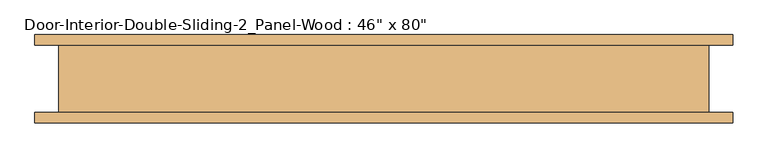
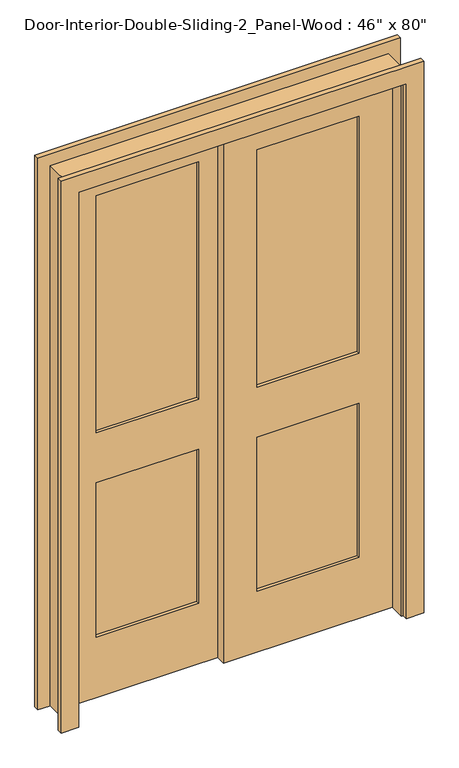
"""IFC4 building model written with IfcOpenShell, lengths in millimetres: door geometry."""

import ifcopenshell
import ifcopenshell.guid

model = None  # the IFC model being written
_history = None  # IfcOwnerHistory: only IFC2X3 demands one
_inside = {}  # id of a spatial element -> (the spatial element, [elements in it])
_under = {}  # id of a project, library or spatial element -> (it, [spatial elements below it])
_declared = {}  # id of a project -> (the project, [libraries it declares])
_typed = {}  # id of a type object -> (the type object, [elements of that type])
_made_of = {}  # id of a material, layer set ... -> (it, [elements and type objects made of it])


def new_model(schema):
    """Start an empty IFC model of exactly this schema.

    Asked for "IFC4X3", IfcOpenShell would pick the latest addendum, in which some entities
    have other attributes; the version numbers below select the first issue.
    IFC2X3 requires an IfcOwnerHistory on every rooted entity: one is made here for all.
    """
    global model, _history
    if schema == "IFC4X3":
        model = ifcopenshell.file(schema_version=(4, 3, 0, 0))
    else:
        model = ifcopenshell.file(schema=schema)
    _inside.clear()
    _under.clear()
    _declared.clear()
    _typed.clear()
    _made_of.clear()
    _history = None
    if model.schema == "IFC2X3":
        org = make("IfcOrganization", Name="unknown")
        user = make(
            "IfcPersonAndOrganization",
            ThePerson=make("IfcPerson", FamilyName="unknown"),
            TheOrganization=org,
        )
        app = make(
            "IfcApplication",
            ApplicationDeveloper=org,
            Version="unknown",
            ApplicationFullName="unknown",
            ApplicationIdentifier="unknown",
        )
        _history = make(
            "IfcOwnerHistory",
            OwningUser=user,
            OwningApplication=app,
            ChangeAction="ADDED",
            CreationDate=0,
        )
    return model


def make(cls, **values):
    """One entity of the class cls with the attributes given. An attribute that is None is left unset."""
    return model.create_entity(
        cls, **{name: value for name, value in values.items() if value is not None}
    )


def rooted(cls, **values):
    """An entity with a GlobalId (a new one), such as an element, a storey or a relation."""
    return make(cls, GlobalId=ifcopenshell.guid.new(), OwnerHistory=_history, **values)


def si_unit(unit_type, name, prefix=None):
    """IfcSIUnit, for example si_unit("LENGTHUNIT", "METRE", prefix="MILLI")."""
    return make("IfcSIUnit", UnitType=unit_type, Prefix=prefix, Name=name)


def assignment(units):
    """IfcUnitAssignment: the units of a project."""
    return None if units is None else make("IfcUnitAssignment", Units=units)


def point(xyz):
    """IfcCartesianPoint."""
    return None if xyz is None else make("IfcCartesianPoint", Coordinates=xyz)


def direction(xyz):
    """IfcDirection."""
    return None if xyz is None else make("IfcDirection", DirectionRatios=xyz)


def frame(location, z_axis=None, x_axis=None):
    """IfcAxis2Placement3D, a coordinate frame: its origin and axes. An axis left out is left unset."""
    return make(
        "IfcAxis2Placement3D",
        Location=point(location),
        Axis=direction(z_axis),
        RefDirection=direction(x_axis),
    )


def origin():
    """The frame at (0, 0, 0) with its axes left unset."""
    return frame((0.0, 0.0, 0.0))


def place(relative_to, where):
    """IfcLocalPlacement: puts the frame where relative to a parent placement (None: the world)."""
    return make(
        "IfcLocalPlacement", PlacementRelTo=relative_to, RelativePlacement=where
    )


def context(
    kind, dimensions, precision=None, world=None, true_north=None, identifier=None
):
    """IfcGeometricRepresentationContext, for example the 3D "Model" context."""
    return make(
        "IfcGeometricRepresentationContext",
        ContextIdentifier=identifier,
        ContextType=kind,
        CoordinateSpaceDimension=dimensions,
        Precision=precision,
        WorldCoordinateSystem=world,
        TrueNorth=true_north,
    )


def project(units=None, contexts=None):
    """IfcProject with its units and contexts."""
    return rooted(
        "IfcProject",
        Name="project",
        RepresentationContexts=contexts,
        UnitsInContext=assignment(units),
    )


def spatial(cls, under=None, at=None, **own):
    """A site, building, storey or space (cls), placed at a placement, below another one or the project."""
    s = rooted(cls, ObjectPlacement=at, **own)
    if under is not None:
        _under.setdefault(under.id(), (under, []))[1].append(s)
    return s


def polyline(points):
    """IfcPolyline through the points."""
    return make("IfcPolyline", Points=[point(p) for p in points])


def outline(outer, holes=None, kind="AREA"):
    """IfcArbitraryClosedProfileDef: a profile drawn as a closed curve; with holes, ...WithVoids."""
    if holes is None:
        return make("IfcArbitraryClosedProfileDef", ProfileType=kind, OuterCurve=outer)
    return make(
        "IfcArbitraryProfileDefWithVoids",
        ProfileType=kind,
        OuterCurve=outer,
        InnerCurves=holes,
    )


def extrude(swept, where, along, depth):
    """IfcExtrudedAreaSolid: the profile swept, set in the frame where, extruded along a direction by depth."""
    return make(
        "IfcExtrudedAreaSolid",
        SweptArea=swept,
        Position=where,
        ExtrudedDirection=direction(along),
        Depth=depth,
    )


def shape(context_of_items, identifier, shape_type, items):
    """IfcShapeRepresentation: the items that make up one representation, for example the "Body"."""
    return make(
        "IfcShapeRepresentation",
        ContextOfItems=context_of_items,
        RepresentationIdentifier=identifier,
        RepresentationType=shape_type,
        Items=items,
    )


def source(mapping_origin, context_of_items, identifier, shape_type, items):
    """IfcRepresentationMap: a shape defined once, which mapped items show again and again."""
    return make(
        "IfcRepresentationMap",
        MappingOrigin=mapping_origin,
        MappedRepresentation=shape(context_of_items, identifier, shape_type, items),
    )


def transform(
    local_origin,
    x_axis=None,
    y_axis=None,
    z_axis=None,
    scale=None,
    scale2=None,
    scale3=None,
    uniform=True,
):
    """IfcCartesianTransformationOperator3D, or its non-uniform kind. x_axis, y_axis, z_axis: its Axis1, 2, 3."""
    if uniform:
        return make(
            "IfcCartesianTransformationOperator3D",
            Axis1=direction(x_axis),
            Axis2=direction(y_axis),
            LocalOrigin=point(local_origin),
            Scale=scale,
            Axis3=direction(z_axis),
        )
    return make(
        "IfcCartesianTransformationOperator3DnonUniform",
        Axis1=direction(x_axis),
        Axis2=direction(y_axis),
        LocalOrigin=point(local_origin),
        Scale=scale,
        Axis3=direction(z_axis),
        Scale2=scale2,
        Scale3=scale3,
    )


def mapped(mapping_source, mapping_target):
    """IfcMappedItem: shows the shape of a source again, moved by a transform."""
    return make(
        "IfcMappedItem", MappingSource=mapping_source, MappingTarget=mapping_target
    )


def made_of(thing, what):
    """Note that an element or type object is made of a material, layer set ...; save() writes the relation."""
    if what is not None:
        _made_of.setdefault(what.id(), (what, []))[1].append(thing)
    return thing


def element(
    cls,
    number,
    at=None,
    inside=None,
    cuts=None,
    type_object=None,
    material=None,
    context=None,
    identifier="Body",
    shape_type=None,
    held_by="IfcProductDefinitionShape",
    body=None,
    shapes=None,
    **own,
):
    """One element of the class cls, such as IfcWall. Its Tag is "e" and its number.

    at: its placement. inside: the storey or other place that contains it. cuts: it is an
    opening in that element (IfcRelVoidsElement). A single representation is given by context,
    identifier, shape_type and body (its items); several are given by shapes. held_by: the class
    of the entity that holds the representations. save() writes the other relations.
    """
    e = rooted(cls, Tag="e%d" % number, ObjectPlacement=at, **own)
    if body is not None:
        shapes = [shape(context, identifier, shape_type, body)]
    if shapes is not None:
        e.Representation = make(held_by, Representations=shapes)
    if inside is not None:
        _inside.setdefault(inside.id(), (inside, []))[1].append(e)
    if cuts is not None:
        rooted(
            "IfcRelVoidsElement", RelatingBuildingElement=cuts, RelatedOpeningElement=e
        )
    if type_object is not None:
        _typed.setdefault(type_object.id(), (type_object, []))[1].append(e)
    return made_of(e, material)


def aggregate(whole, parts):
    """IfcRelAggregates: a whole, such as a stair, and the parts it consists of."""
    return rooted("IfcRelAggregates", RelatingObject=whole, RelatedObjects=parts)


def save(model, path):
    """Write the relations noted so far, then the file.

    IfcRelAggregates (storeys below a building ...), IfcRelContainedInSpatialStructure (elements
    in a storey), IfcRelDefinesByType, IfcRelAssociatesMaterial and IfcRelDeclares: one each for
    every whole, place, type object, material and project.
    """
    for whole, parts in _under.values():
        aggregate(whole, parts)
    for where, things in _inside.values():
        rooted(
            "IfcRelContainedInSpatialStructure",
            RelatedElements=things,
            RelatingStructure=where,
        )
    for kind, things in _typed.values():
        rooted("IfcRelDefinesByType", RelatedObjects=things, RelatingType=kind)
    for what, things in _made_of.values():
        rooted("IfcRelAssociatesMaterial", RelatedObjects=things, RelatingMaterial=what)
    for by, libraries in _declared.values():
        rooted("IfcRelDeclares", RelatingContext=by, RelatedDefinitions=libraries)
    model.write(path)


def door_0fd0fe05(model_context):
    return source(origin(), model_context, "Body", "SweptSolid", [
        extrude(outline(polyline([(463.55, 2.1166667), (95.25, 2.1166667), (95.25, 13.7583333), (463.55, 13.7583333), (463.55, 2.1166667)])), frame((0.0, 0.0, 1009.65), z_axis=(0.0, 0.0, 1.0), x_axis=(1.0, 0.0, 0.0)), (0.0, 0.0, 1.0), 903.2875),
        extrude(outline(polyline([(463.55, 2.1166667), (95.25, 2.1166667), (95.25, 13.7583333), (463.55, 13.7583333), (463.55, 2.1166667)])), frame((0.0, 0.0, 231.775), z_axis=(0.0, 0.0, 1.0), x_axis=(1.0, 0.0, 0.0)), (0.0, 0.0, 1.0), 587.375),
        extrude(outline(polyline([(2032.0, -25.4), (0.0, -25.4), (0.0, 584.2), (2032.0, 584.2), (2032.0, -25.4)]), holes=[polyline([(1912.9375, 95.25), (1912.9375, 463.55), (1009.65, 463.55), (1009.65, 95.25), (1912.9375, 95.25)]), polyline([(819.15, 95.25), (819.15, 463.55), (231.775, 463.55), (231.775, 95.25), (819.15, 95.25)])]), frame((0.0, -9.525, 0.0), z_axis=(0.0, 1.0, 0.0), x_axis=(0.0, 0.0, 1.0)), (0.0, 0.0, 1.0), 34.925),
        extrude(outline(polyline([(-95.25, 37.0416667), (-463.55, 37.0416667), (-463.55, 48.6833333), (-95.25, 48.6833333), (-95.25, 37.0416667)])), frame((0.0, 0.0, 1009.65), z_axis=(0.0, 0.0, 1.0), x_axis=(1.0, 0.0, 0.0)), (0.0, 0.0, 1.0), 903.2875),
        extrude(outline(polyline([(-95.25, 37.0416667), (-463.55, 37.0416667), (-463.55, 48.6833333), (-95.25, 48.6833333), (-95.25, 37.0416667)])), frame((0.0, 0.0, 231.775), z_axis=(0.0, 0.0, 1.0), x_axis=(1.0, 0.0, 0.0)), (0.0, 0.0, 1.0), 587.375),
        extrude(outline(polyline([(2032.0, -584.2), (0.0, -584.2), (0.0, 25.4), (2032.0, 25.4), (2032.0, -584.2)]), holes=[polyline([(1912.9375, -463.55), (1912.9375, -95.25), (1009.65, -95.25), (1009.65, -463.55), (1912.9375, -463.55)]), polyline([(819.15, -463.55), (819.15, -95.25), (231.775, -95.25), (231.775, -463.55), (819.15, -463.55)])]), frame((0.0, 25.4, 0.0), z_axis=(0.0, 1.0, 0.0), x_axis=(0.0, 0.0, 1.0)), (0.0, 0.0, 1.0), 34.925),
        extrude(outline(polyline([(0.0, 584.2), (0.0, 609.6), (2057.4, 609.6), (2057.4, -609.6), (0.0, -609.6), (0.0, -584.2), (2032.0, -584.2), (2032.0, 584.2), (0.0, 584.2)])), frame((0.0, -66.675, 0.0), z_axis=(0.0, 1.0, 0.0), x_axis=(0.0, 0.0, 1.0)), (0.0, 0.0, 1.0), 127.0),
        extrude(outline(polyline([(0.0, 590.55), (0.0, 654.05), (2101.85, 654.05), (2101.85, -654.05), (0.0, -654.05), (0.0, -590.55), (2038.35, -590.55), (2038.35, 590.55), (0.0, 590.55)])), frame((0.0, -85.725, 0.0), z_axis=(0.0, 1.0, 0.0), x_axis=(0.0, 0.0, 1.0)), (0.0, 0.0, 1.0), 19.05),
        extrude(outline(polyline([(0.0, 590.55), (0.0, 654.05), (2101.85, 654.05), (2101.85, -654.05), (0.0, -654.05), (0.0, -590.55), (2038.35, -590.55), (2038.35, 590.55), (0.0, 590.55)])), frame((0.0, 60.325, 0.0), z_axis=(0.0, 1.0, 0.0), x_axis=(0.0, 0.0, 1.0)), (0.0, 0.0, 1.0), 19.05),
    ])


if __name__ == "__main__":
    model = new_model("IFC4")
    model_context = context("Model", 3, world=origin())
    ifc_project = project(units=[si_unit("LENGTHUNIT", "METRE", prefix="MILLI")], contexts=[model_context])
    site = spatial("IfcSite", under=ifc_project)
    building = spatial("IfcBuilding", under=site)
    placement = place(None, origin())
    door_shape = door_0fd0fe05(model_context)
    element("IfcDoor", 1, ObjectType="Door-Interior-Double-Sliding-2_Panel-Wood : 46\" x 80\"", at=placement, inside=building, context=model_context, shape_type="MappedRepresentation", body=[
        mapped(door_shape, transform((0.0, 0.0, 0.0), x_axis=(1.0, 0.0, 0.0), y_axis=(0.0, 1.0, 0.0), z_axis=(0.0, 0.0, 1.0))),
    ])
    save(model, "model.ifc")

# Revit data of these elements
# Type "Door-Interior-Double-Sliding-2_Panel-Wood : 46\" x 80\""
#   Type Mark = "26"
#   Assembly Code = "C1020300"
#   Analytic Construction = "Wooden"
#   Top Rail = 0' - 4 11/16"
#   Thickness = 0' - 1 3/8"
#   Thermal Resistance (R) = 2.5876 (h·ft²·°F)/BTU
#   Stiles = 0' - 4 3/4"
#   Rough Width = 4' - 0"
#   Rough Height = 6' - 9"
#   Lock Rail = 0' - 7 1/2"
#   Height = 6' - 8"
#   Width = 3' - 10"
#   Heat Transfer Coefficient (U) = 0.3865 BTU/(h·ft²·°F)
#   Bottom Rail = 0' - 9 1/8"
#   Trim Material = Cherry
#   Panel Material = Cherry
#   Frame Material = Cherry
#   Visual Light Transmittance = 0
#   Solar Heat Gain Coefficient = 0
#   Wall Closure = (empty or 0)
#   Function = (empty or 0)
# Element 1 (IfcDoor, "Door-Interior-Double-Sliding-2_Panel-Wood : 46\" x 80\"")
#   Materials on its faces: "Cherry"
# Materials
#   "Cherry": class "Wood", colour RGB 226 177 128, transparency 0, Description = "Prunus Serotina", Cost = 0
